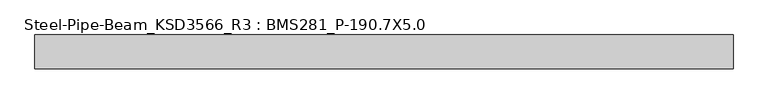
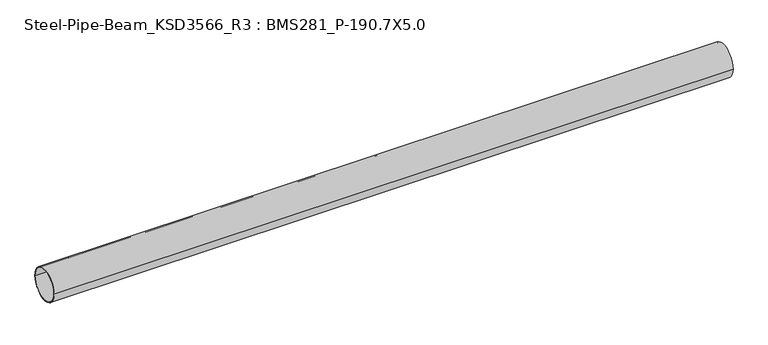
"""IFC4 building model written with IfcOpenShell, lengths in millimetres: member geometry, Steel-Pipe-Beam_KSD3566_R3 : BMS281_P-190.7X5.0."""

import ifcopenshell
import ifcopenshell.guid

model = None  # the IFC model being written
_history = None  # IfcOwnerHistory: only IFC2X3 demands one
_inside = {}  # id of a spatial element -> (the spatial element, [elements in it])
_under = {}  # id of a project, library or spatial element -> (it, [spatial elements below it])
_declared = {}  # id of a project -> (the project, [libraries it declares])
_typed = {}  # id of a type object -> (the type object, [elements of that type])
_made_of = {}  # id of a material, layer set ... -> (it, [elements and type objects made of it])


def new_model(schema):
    """Start an empty IFC model of exactly this schema.

    Asked for "IFC4X3", IfcOpenShell would pick the latest addendum, in which some entities
    have other attributes; the version numbers below select the first issue.
    IFC2X3 requires an IfcOwnerHistory on every rooted entity: one is made here for all.
    """
    global model, _history
    if schema == "IFC4X3":
        model = ifcopenshell.file(schema_version=(4, 3, 0, 0))
    else:
        model = ifcopenshell.file(schema=schema)
    _inside.clear()
    _under.clear()
    _declared.clear()
    _typed.clear()
    _made_of.clear()
    _history = None
    if model.schema == "IFC2X3":
        org = make("IfcOrganization", Name="unknown")
        user = make(
            "IfcPersonAndOrganization",
            ThePerson=make("IfcPerson", FamilyName="unknown"),
            TheOrganization=org,
        )
        app = make(
            "IfcApplication",
            ApplicationDeveloper=org,
            Version="unknown",
            ApplicationFullName="unknown",
            ApplicationIdentifier="unknown",
        )
        _history = make(
            "IfcOwnerHistory",
            OwningUser=user,
            OwningApplication=app,
            ChangeAction="ADDED",
            CreationDate=0,
        )
    return model


def make(cls, **values):
    """One entity of the class cls with the attributes given. An attribute that is None is left unset."""
    return model.create_entity(
        cls, **{name: value for name, value in values.items() if value is not None}
    )


def rooted(cls, **values):
    """An entity with a GlobalId (a new one), such as an element, a storey or a relation."""
    return make(cls, GlobalId=ifcopenshell.guid.new(), OwnerHistory=_history, **values)


def si_unit(unit_type, name, prefix=None):
    """IfcSIUnit, for example si_unit("LENGTHUNIT", "METRE", prefix="MILLI")."""
    return make("IfcSIUnit", UnitType=unit_type, Prefix=prefix, Name=name)


def assignment(units):
    """IfcUnitAssignment: the units of a project."""
    return None if units is None else make("IfcUnitAssignment", Units=units)


def point(xyz):
    """IfcCartesianPoint."""
    return None if xyz is None else make("IfcCartesianPoint", Coordinates=xyz)


def direction(xyz):
    """IfcDirection."""
    return None if xyz is None else make("IfcDirection", DirectionRatios=xyz)


def frame(location, z_axis=None, x_axis=None):
    """IfcAxis2Placement3D, a coordinate frame: its origin and axes. An axis left out is left unset."""
    return make(
        "IfcAxis2Placement3D",
        Location=point(location),
        Axis=direction(z_axis),
        RefDirection=direction(x_axis),
    )


def frame_2d(location, x_axis=None):
    """IfcAxis2Placement2D, a coordinate frame in the plane: its origin and x axis."""
    return make(
        "IfcAxis2Placement2D", Location=point(location), RefDirection=direction(x_axis)
    )


def origin():
    """The frame at (0, 0, 0) with its axes left unset."""
    return frame((0.0, 0.0, 0.0))


def origin_2d():
    """The frame at (0, 0) in the plane with its x axis left unset."""
    return frame_2d((0.0, 0.0))


def place(relative_to, where):
    """IfcLocalPlacement: puts the frame where relative to a parent placement (None: the world)."""
    return make(
        "IfcLocalPlacement", PlacementRelTo=relative_to, RelativePlacement=where
    )


def context(
    kind, dimensions, precision=None, world=None, true_north=None, identifier=None
):
    """IfcGeometricRepresentationContext, for example the 3D "Model" context."""
    return make(
        "IfcGeometricRepresentationContext",
        ContextIdentifier=identifier,
        ContextType=kind,
        CoordinateSpaceDimension=dimensions,
        Precision=precision,
        WorldCoordinateSystem=world,
        TrueNorth=true_north,
    )


def project(units=None, contexts=None):
    """IfcProject with its units and contexts."""
    return rooted(
        "IfcProject",
        Name="project",
        RepresentationContexts=contexts,
        UnitsInContext=assignment(units),
    )


def spatial(cls, under=None, at=None, **own):
    """A site, building, storey or space (cls), placed at a placement, below another one or the project."""
    s = rooted(cls, ObjectPlacement=at, **own)
    if under is not None:
        _under.setdefault(under.id(), (under, []))[1].append(s)
    return s


def circle_curve(where, radius):
    """IfcCircle in the frame where."""
    return make("IfcCircle", Position=where, Radius=radius)


def trimmed(basis, trim1, trim2, sense, master):
    """IfcTrimmedCurve: the piece of a basis curve between two trims."""
    return make(
        "IfcTrimmedCurve",
        BasisCurve=basis,
        Trim1=trim1,
        Trim2=trim2,
        SenseAgreement=sense,
        MasterRepresentation=master,
    )


def segment(curve, same_sense, transition):
    """IfcCompositeCurveSegment."""
    return make(
        "IfcCompositeCurveSegment",
        Transition=transition,
        SameSense=same_sense,
        ParentCurve=curve,
    )


def composite_curve(segments, self_intersect=None):
    """IfcCompositeCurve: segments joined end to end."""
    return make("IfcCompositeCurve", Segments=segments, SelfIntersect=self_intersect)


def outline(outer, holes=None, kind="AREA"):
    """IfcArbitraryClosedProfileDef: a profile drawn as a closed curve; with holes, ...WithVoids."""
    if holes is None:
        return make("IfcArbitraryClosedProfileDef", ProfileType=kind, OuterCurve=outer)
    return make(
        "IfcArbitraryProfileDefWithVoids",
        ProfileType=kind,
        OuterCurve=outer,
        InnerCurves=holes,
    )


def extrude(swept, where, along, depth):
    """IfcExtrudedAreaSolid: the profile swept, set in the frame where, extruded along a direction by depth."""
    return make(
        "IfcExtrudedAreaSolid",
        SweptArea=swept,
        Position=where,
        ExtrudedDirection=direction(along),
        Depth=depth,
    )


def shape(context_of_items, identifier, shape_type, items):
    """IfcShapeRepresentation: the items that make up one representation, for example the "Body"."""
    return make(
        "IfcShapeRepresentation",
        ContextOfItems=context_of_items,
        RepresentationIdentifier=identifier,
        RepresentationType=shape_type,
        Items=items,
    )


def source(mapping_origin, context_of_items, identifier, shape_type, items):
    """IfcRepresentationMap: a shape defined once, which mapped items show again and again."""
    return make(
        "IfcRepresentationMap",
        MappingOrigin=mapping_origin,
        MappedRepresentation=shape(context_of_items, identifier, shape_type, items),
    )


def transform(
    local_origin,
    x_axis=None,
    y_axis=None,
    z_axis=None,
    scale=None,
    scale2=None,
    scale3=None,
    uniform=True,
):
    """IfcCartesianTransformationOperator3D, or its non-uniform kind. x_axis, y_axis, z_axis: its Axis1, 2, 3."""
    if uniform:
        return make(
            "IfcCartesianTransformationOperator3D",
            Axis1=direction(x_axis),
            Axis2=direction(y_axis),
            LocalOrigin=point(local_origin),
            Scale=scale,
            Axis3=direction(z_axis),
        )
    return make(
        "IfcCartesianTransformationOperator3DnonUniform",
        Axis1=direction(x_axis),
        Axis2=direction(y_axis),
        LocalOrigin=point(local_origin),
        Scale=scale,
        Axis3=direction(z_axis),
        Scale2=scale2,
        Scale3=scale3,
    )


def mapped(mapping_source, mapping_target):
    """IfcMappedItem: shows the shape of a source again, moved by a transform."""
    return make(
        "IfcMappedItem", MappingSource=mapping_source, MappingTarget=mapping_target
    )


def made_of(thing, what):
    """Note that an element or type object is made of a material, layer set ...; save() writes the relation."""
    if what is not None:
        _made_of.setdefault(what.id(), (what, []))[1].append(thing)
    return thing


def element(
    cls,
    number,
    at=None,
    inside=None,
    cuts=None,
    type_object=None,
    material=None,
    context=None,
    identifier="Body",
    shape_type=None,
    held_by="IfcProductDefinitionShape",
    body=None,
    shapes=None,
    **own,
):
    """One element of the class cls, such as IfcWall. Its Tag is "e" and its number.

    at: its placement. inside: the storey or other place that contains it. cuts: it is an
    opening in that element (IfcRelVoidsElement). A single representation is given by context,
    identifier, shape_type and body (its items); several are given by shapes. held_by: the class
    of the entity that holds the representations. save() writes the other relations.
    """
    e = rooted(cls, Tag="e%d" % number, ObjectPlacement=at, **own)
    if body is not None:
        shapes = [shape(context, identifier, shape_type, body)]
    if shapes is not None:
        e.Representation = make(held_by, Representations=shapes)
    if inside is not None:
        _inside.setdefault(inside.id(), (inside, []))[1].append(e)
    if cuts is not None:
        rooted(
            "IfcRelVoidsElement", RelatingBuildingElement=cuts, RelatedOpeningElement=e
        )
    if type_object is not None:
        _typed.setdefault(type_object.id(), (type_object, []))[1].append(e)
    return made_of(e, material)


def aggregate(whole, parts):
    """IfcRelAggregates: a whole, such as a stair, and the parts it consists of."""
    return rooted("IfcRelAggregates", RelatingObject=whole, RelatedObjects=parts)


def save(model, path):
    """Write the relations noted so far, then the file.

    IfcRelAggregates (storeys below a building ...), IfcRelContainedInSpatialStructure (elements
    in a storey), IfcRelDefinesByType, IfcRelAssociatesMaterial and IfcRelDeclares: one each for
    every whole, place, type object, material and project.
    """
    for whole, parts in _under.values():
        aggregate(whole, parts)
    for where, things in _inside.values():
        rooted(
            "IfcRelContainedInSpatialStructure",
            RelatedElements=things,
            RelatingStructure=where,
        )
    for kind, things in _typed.values():
        rooted("IfcRelDefinesByType", RelatedObjects=things, RelatingType=kind)
    for what, things in _made_of.values():
        rooted("IfcRelAssociatesMaterial", RelatedObjects=things, RelatingMaterial=what)
    for by, libraries in _declared.values():
        rooted("IfcRelDeclares", RelatingContext=by, RelatedDefinitions=libraries)
    model.write(path)


def steel_pipe_beam_ksd3566_r3_bms281_p_190_7x5_0_c9e99e3d(model_context):
    return source(origin(), model_context, "Body", "SweptSolid", [
        extrude(outline(composite_curve([segment(trimmed(circle_curve(origin_2d(), 95.35), [point((95.35, 0.0))], [point((-95.35, 0.0))], False, "CARTESIAN"), True, "CONTINUOUS"), segment(trimmed(circle_curve(origin_2d(), 95.35), [point((-95.35, 0.0))], [point((95.35, 0.0))], False, "CARTESIAN"), True, "CONTINUOUS")], self_intersect=False), holes=[composite_curve([segment(trimmed(circle_curve(origin_2d(), 90.35), [point((-90.35, 0.0))], [point((90.35, 0.0))], True, "CARTESIAN"), True, "CONTINUOUS"), segment(trimmed(circle_curve(origin_2d(), 90.35), [point((90.35, 0.0))], [point((-90.35, 0.0))], True, "CARTESIAN"), True, "CONTINUOUS")], self_intersect=False)]), frame((-1979.4197206, 0.0, 0.0), z_axis=(1.0, 0.0, 0.0), x_axis=(0.0, 1.0, 0.0)), (0.0, 0.0, 1.0), 3944.9083215),
    ])


if __name__ == "__main__":
    model = new_model("IFC4")
    model_context = context("Model", 3, world=origin())
    ifc_project = project(units=[si_unit("LENGTHUNIT", "METRE", prefix="MILLI")], contexts=[model_context])
    site = spatial("IfcSite", under=ifc_project)
    building = spatial("IfcBuilding", under=site)
    placement = place(None, origin())
    steel_pipe_beam_ksd3566_r3_bms281_p_190_7x5_0_shape = steel_pipe_beam_ksd3566_r3_bms281_p_190_7x5_0_c9e99e3d(model_context)
    element("IfcMember", 1, ObjectType="Steel-Pipe-Beam_KSD3566_R3 : BMS281_P-190.7X5.0", at=placement, inside=building, context=model_context, shape_type="MappedRepresentation", body=[
        mapped(steel_pipe_beam_ksd3566_r3_bms281_p_190_7x5_0_shape, transform((0.0, 0.0, 0.0), x_axis=(1.0, 0.0, 0.0), y_axis=(0.0, 1.0, 0.0), z_axis=(0.0, 0.0, 1.0))),
    ])
    save(model, "model.ifc")

# Revit data of these elements
# Type "Steel-Pipe-Beam_KSD3566_R3 : BMS281_P-190.7X5.0"
#   Keynote = "P-190.7X5.0"
#   SteelWeight = "Light"
#   t = 0.0050 m
#   Surface Area = 0.599102 m²/m
#   Section Area = 29.1697 cm²
#   Mass per Unit Length = 22.8982 kg/m
#   Length [instance default] = 1.5000 m
#   D = 0.1907 m
#   hec_material4 [instance default] = none
#   hec_material3 [instance default] = none
#   hec_material2 [instance default] = none
#   hec_material1 [instance default] = none
#   Structural Material [instance default] = Steel, 45-345
#   Assembly Code = ""
# Element 1 (IfcMember, "Steel-Pipe-Beam_KSD3566_R3 : BMS281_P-190.7X5.0")
#   Structural Material = none
# Materials
#   "Steel, 45-345": class "Metal", colour RGB 189 187 185, transparency 0, Description = "Steel 345 MPa", Cost = 0
